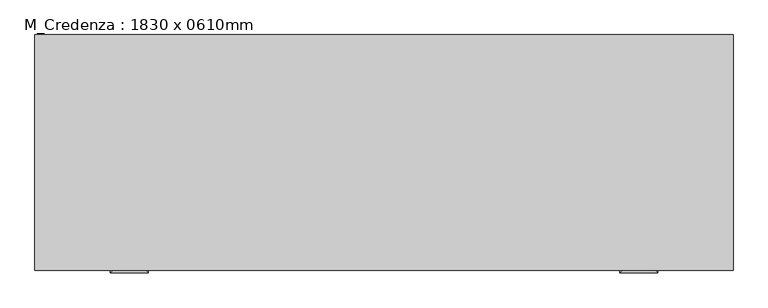
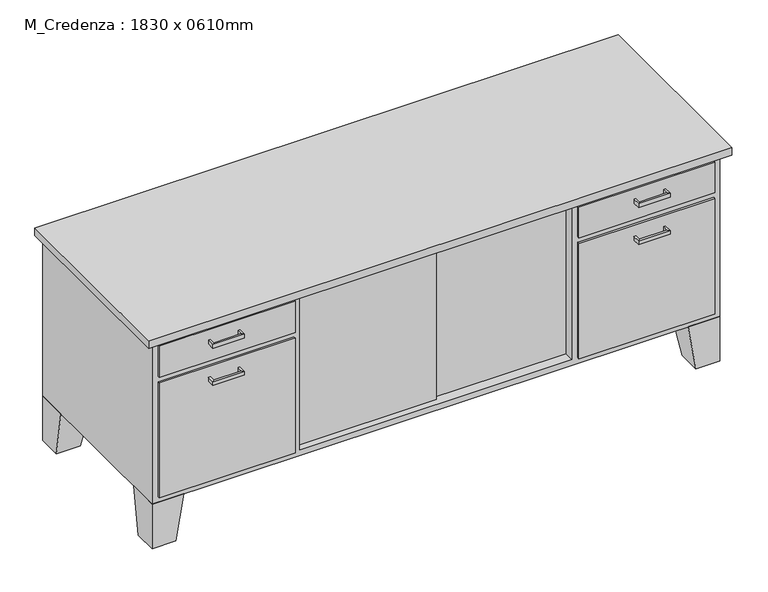
"""IFC4 building model written with IfcOpenShell, lengths in millimetres: furniture geometry, M_Credenza : 1830 x 0610mm."""

import ifcopenshell
import ifcopenshell.guid

model = None  # the IFC model being written
_history = None  # IfcOwnerHistory: only IFC2X3 demands one
_inside = {}  # id of a spatial element -> (the spatial element, [elements in it])
_under = {}  # id of a project, library or spatial element -> (it, [spatial elements below it])
_declared = {}  # id of a project -> (the project, [libraries it declares])
_typed = {}  # id of a type object -> (the type object, [elements of that type])
_made_of = {}  # id of a material, layer set ... -> (it, [elements and type objects made of it])


def new_model(schema):
    """Start an empty IFC model of exactly this schema.

    Asked for "IFC4X3", IfcOpenShell would pick the latest addendum, in which some entities
    have other attributes; the version numbers below select the first issue.
    IFC2X3 requires an IfcOwnerHistory on every rooted entity: one is made here for all.
    """
    global model, _history
    if schema == "IFC4X3":
        model = ifcopenshell.file(schema_version=(4, 3, 0, 0))
    else:
        model = ifcopenshell.file(schema=schema)
    _inside.clear()
    _under.clear()
    _declared.clear()
    _typed.clear()
    _made_of.clear()
    _history = None
    if model.schema == "IFC2X3":
        org = make("IfcOrganization", Name="unknown")
        user = make(
            "IfcPersonAndOrganization",
            ThePerson=make("IfcPerson", FamilyName="unknown"),
            TheOrganization=org,
        )
        app = make(
            "IfcApplication",
            ApplicationDeveloper=org,
            Version="unknown",
            ApplicationFullName="unknown",
            ApplicationIdentifier="unknown",
        )
        _history = make(
            "IfcOwnerHistory",
            OwningUser=user,
            OwningApplication=app,
            ChangeAction="ADDED",
            CreationDate=0,
        )
    return model


def make(cls, **values):
    """One entity of the class cls with the attributes given. An attribute that is None is left unset."""
    return model.create_entity(
        cls, **{name: value for name, value in values.items() if value is not None}
    )


def rooted(cls, **values):
    """An entity with a GlobalId (a new one), such as an element, a storey or a relation."""
    return make(cls, GlobalId=ifcopenshell.guid.new(), OwnerHistory=_history, **values)


def si_unit(unit_type, name, prefix=None):
    """IfcSIUnit, for example si_unit("LENGTHUNIT", "METRE", prefix="MILLI")."""
    return make("IfcSIUnit", UnitType=unit_type, Prefix=prefix, Name=name)


def assignment(units):
    """IfcUnitAssignment: the units of a project."""
    return None if units is None else make("IfcUnitAssignment", Units=units)


def point(xyz):
    """IfcCartesianPoint."""
    return None if xyz is None else make("IfcCartesianPoint", Coordinates=xyz)


def direction(xyz):
    """IfcDirection."""
    return None if xyz is None else make("IfcDirection", DirectionRatios=xyz)


def frame(location, z_axis=None, x_axis=None):
    """IfcAxis2Placement3D, a coordinate frame: its origin and axes. An axis left out is left unset."""
    return make(
        "IfcAxis2Placement3D",
        Location=point(location),
        Axis=direction(z_axis),
        RefDirection=direction(x_axis),
    )


def origin():
    """The frame at (0, 0, 0) with its axes left unset."""
    return frame((0.0, 0.0, 0.0))


def place(relative_to, where):
    """IfcLocalPlacement: puts the frame where relative to a parent placement (None: the world)."""
    return make(
        "IfcLocalPlacement", PlacementRelTo=relative_to, RelativePlacement=where
    )


def context(
    kind, dimensions, precision=None, world=None, true_north=None, identifier=None
):
    """IfcGeometricRepresentationContext, for example the 3D "Model" context."""
    return make(
        "IfcGeometricRepresentationContext",
        ContextIdentifier=identifier,
        ContextType=kind,
        CoordinateSpaceDimension=dimensions,
        Precision=precision,
        WorldCoordinateSystem=world,
        TrueNorth=true_north,
    )


def project(units=None, contexts=None):
    """IfcProject with its units and contexts."""
    return rooted(
        "IfcProject",
        Name="project",
        RepresentationContexts=contexts,
        UnitsInContext=assignment(units),
    )


def spatial(cls, under=None, at=None, **own):
    """A site, building, storey or space (cls), placed at a placement, below another one or the project."""
    s = rooted(cls, ObjectPlacement=at, **own)
    if under is not None:
        _under.setdefault(under.id(), (under, []))[1].append(s)
    return s


def polyline(points):
    """IfcPolyline through the points."""
    return make("IfcPolyline", Points=[point(p) for p in points])


def outline(outer, holes=None, kind="AREA"):
    """IfcArbitraryClosedProfileDef: a profile drawn as a closed curve; with holes, ...WithVoids."""
    if holes is None:
        return make("IfcArbitraryClosedProfileDef", ProfileType=kind, OuterCurve=outer)
    return make(
        "IfcArbitraryProfileDefWithVoids",
        ProfileType=kind,
        OuterCurve=outer,
        InnerCurves=holes,
    )


def extrude(swept, where, along, depth):
    """IfcExtrudedAreaSolid: the profile swept, set in the frame where, extruded along a direction by depth."""
    return make(
        "IfcExtrudedAreaSolid",
        SweptArea=swept,
        Position=where,
        ExtrudedDirection=direction(along),
        Depth=depth,
    )


def faces_of(points, faces, orient=None, outer=None):
    """IfcFace entities. A face is a list of loops; a loop is a list of indices into points, from 0.

    orient and outer hold one flag for each loop. By default every Orientation is true, the
    first loop of a face is its IfcFaceOuterBound and the others are IfcFaceBound.
    """
    made = []
    for i, loops in enumerate(faces):
        bounds = []
        for j, loop in enumerate(loops):
            is_outer = j == 0 if outer is None else outer[i][j]
            bounds.append(
                make(
                    "IfcFaceOuterBound" if is_outer else "IfcFaceBound",
                    Bound=make("IfcPolyLoop", Polygon=[points[k] for k in loop]),
                    Orientation=True if orient is None else orient[i][j],
                )
            )
        made.append(make("IfcFace", Bounds=bounds))
    return made


def faceted_brep(points, faces, orient=None, outer=None, voids=None):
    """IfcFacetedBrep: a solid bounded by flat faces; with voids (closed shells), ...WithVoids."""
    shared = [point(p) for p in points]
    hull = make("IfcClosedShell", CfsFaces=faces_of(shared, faces, orient, outer))
    if voids is None:
        return make("IfcFacetedBrep", Outer=hull)
    return make(
        "IfcFacetedBrepWithVoids",
        Outer=hull,
        Voids=[
            make(cls, CfsFaces=faces_of(shared, fs, o, b)) for cls, fs, o, b in voids
        ],
    )


def shape(context_of_items, identifier, shape_type, items):
    """IfcShapeRepresentation: the items that make up one representation, for example the "Body"."""
    return make(
        "IfcShapeRepresentation",
        ContextOfItems=context_of_items,
        RepresentationIdentifier=identifier,
        RepresentationType=shape_type,
        Items=items,
    )


def source(mapping_origin, context_of_items, identifier, shape_type, items):
    """IfcRepresentationMap: a shape defined once, which mapped items show again and again."""
    return make(
        "IfcRepresentationMap",
        MappingOrigin=mapping_origin,
        MappedRepresentation=shape(context_of_items, identifier, shape_type, items),
    )


def transform(
    local_origin,
    x_axis=None,
    y_axis=None,
    z_axis=None,
    scale=None,
    scale2=None,
    scale3=None,
    uniform=True,
):
    """IfcCartesianTransformationOperator3D, or its non-uniform kind. x_axis, y_axis, z_axis: its Axis1, 2, 3."""
    if uniform:
        return make(
            "IfcCartesianTransformationOperator3D",
            Axis1=direction(x_axis),
            Axis2=direction(y_axis),
            LocalOrigin=point(local_origin),
            Scale=scale,
            Axis3=direction(z_axis),
        )
    return make(
        "IfcCartesianTransformationOperator3DnonUniform",
        Axis1=direction(x_axis),
        Axis2=direction(y_axis),
        LocalOrigin=point(local_origin),
        Scale=scale,
        Axis3=direction(z_axis),
        Scale2=scale2,
        Scale3=scale3,
    )


def mapped(mapping_source, mapping_target):
    """IfcMappedItem: shows the shape of a source again, moved by a transform."""
    return make(
        "IfcMappedItem", MappingSource=mapping_source, MappingTarget=mapping_target
    )


def made_of(thing, what):
    """Note that an element or type object is made of a material, layer set ...; save() writes the relation."""
    if what is not None:
        _made_of.setdefault(what.id(), (what, []))[1].append(thing)
    return thing


def element(
    cls,
    number,
    at=None,
    inside=None,
    cuts=None,
    type_object=None,
    material=None,
    context=None,
    identifier="Body",
    shape_type=None,
    held_by="IfcProductDefinitionShape",
    body=None,
    shapes=None,
    **own,
):
    """One element of the class cls, such as IfcWall. Its Tag is "e" and its number.

    at: its placement. inside: the storey or other place that contains it. cuts: it is an
    opening in that element (IfcRelVoidsElement). A single representation is given by context,
    identifier, shape_type and body (its items); several are given by shapes. held_by: the class
    of the entity that holds the representations. save() writes the other relations.
    """
    e = rooted(cls, Tag="e%d" % number, ObjectPlacement=at, **own)
    if body is not None:
        shapes = [shape(context, identifier, shape_type, body)]
    if shapes is not None:
        e.Representation = make(held_by, Representations=shapes)
    if inside is not None:
        _inside.setdefault(inside.id(), (inside, []))[1].append(e)
    if cuts is not None:
        rooted(
            "IfcRelVoidsElement", RelatingBuildingElement=cuts, RelatedOpeningElement=e
        )
    if type_object is not None:
        _typed.setdefault(type_object.id(), (type_object, []))[1].append(e)
    return made_of(e, material)


def aggregate(whole, parts):
    """IfcRelAggregates: a whole, such as a stair, and the parts it consists of."""
    return rooted("IfcRelAggregates", RelatingObject=whole, RelatedObjects=parts)


def save(model, path):
    """Write the relations noted so far, then the file.

    IfcRelAggregates (storeys below a building ...), IfcRelContainedInSpatialStructure (elements
    in a storey), IfcRelDefinesByType, IfcRelAssociatesMaterial and IfcRelDeclares: one each for
    every whole, place, type object, material and project.
    """
    for whole, parts in _under.values():
        aggregate(whole, parts)
    for where, things in _inside.values():
        rooted(
            "IfcRelContainedInSpatialStructure",
            RelatedElements=things,
            RelatingStructure=where,
        )
    for kind, things in _typed.values():
        rooted("IfcRelDefinesByType", RelatedObjects=things, RelatingType=kind)
    for what, things in _made_of.values():
        rooted("IfcRelAssociatesMaterial", RelatedObjects=things, RelatingMaterial=what)
    for by, libraries in _declared.values():
        rooted("IfcRelDeclares", RelatingContext=by, RelatedDefinitions=libraries)
    model.write(path)


def m_credenza_1830_x_0610mm_1080a9db(model_context):
    return source(origin(), model_context, "Body", "SolidModel", [
        extrude(outline(polyline([(532.0023176, -267.0714583), (46.8442623, -267.0714583), (46.8442623, -254.7714583), (532.0023176, -254.7714583), (532.0023176, -267.0714583)])), frame((0.0, 0.0, 171.45), z_axis=(0.0, 0.0, 1.0), x_axis=(1.0, 0.0, 0.0)), (0.0, 0.0, 1.0), 518.1),
        extrude(outline(polyline([(73.6254475, -279.7714583), (-378.9057377, -279.7714583), (-378.9057377, -267.0714583), (73.6254475, -267.0714583), (73.6254475, -279.7714583)])), frame((0.0, 0.0, 171.45), z_axis=(0.0, 0.0, 1.0), x_axis=(1.0, 0.0, 0.0)), (0.0, 0.0, 1.0), 518.1),
        faceted_brep([(872.9442623, 309.5803279, 152.4), (872.9442623, 207.9803279, 152.4), (974.5442623, 207.9803279, 152.4), (974.5442623, 309.5803279, 152.4), (898.3442623, 309.5803279, 0.0), (974.5442623, 309.5803279, 0.0), (974.5442623, 233.3803279, 0.0), (898.3442623, 233.3803279, 0.0)], [[[0, 1, 2, 3]], [[4, 5, 6, 7]], [[4, 7, 1, 0]], [[7, 6, 2, 1]], [[6, 5, 3, 2]], [[5, 4, 0, 3]]]),
        extrude(outline(polyline([(955.4942623, -306.3696721), (517.0442623, -306.3696721), (517.0442623, -300.0196721), (955.4942623, -300.0196721), (955.4942623, -306.3696721)])), frame((0.0, 0.0, 584.2), z_axis=(0.0, 0.0, 1.0), x_axis=(1.0, 0.0, 0.0)), (0.0, 0.0, 1.0), 105.35),
        extrude(outline(polyline([(955.4942623, -306.3696721), (517.0442623, -306.3696721), (517.0442623, -300.0196721), (955.4942623, -300.0196721), (955.4942623, -306.3696721)])), frame((0.0, 0.0, 171.45), z_axis=(0.0, 0.0, 1.0), x_axis=(1.0, 0.0, 0.0)), (0.0, 0.0, 1.0), 393.7),
        extrude(outline(polyline([(-397.9557377, -306.7696721), (-836.4057377, -306.7696721), (-836.4057377, -300.4196721), (-397.9557377, -300.4196721), (-397.9557377, -306.7696721)])), frame((0.0, 0.0, 581.6), z_axis=(0.0, 0.0, 1.0), x_axis=(1.0, 0.0, 0.0)), (0.0, 0.0, 1.0), 107.95),
        extrude(outline(polyline([(-397.9557377, -306.7696721), (-836.4057377, -306.7696721), (-836.4057377, -300.4196721), (-397.9557377, -300.4196721), (-397.9557377, -306.7696721)])), frame((0.0, 0.0, 171.45), z_axis=(0.0, 0.0, 1.0), x_axis=(1.0, 0.0, 0.0)), (0.0, 0.0, 1.0), 391.1),
        faceted_brep([(-753.8557377, -300.4196721, 152.4), (-753.8557377, -198.8196721, 152.4), (-855.4557377, -198.8196721, 152.4), (-855.4557377, -300.4196721, 152.4), (-779.2557377, -300.4196721, 0.0), (-855.4557377, -300.4196721, 0.0), (-855.4557377, -224.2196721, 0.0), (-779.2557377, -224.2196721, 0.0)], [[[0, 1, 2, 3]], [[4, 5, 6, 7]], [[4, 7, 1, 0]], [[7, 6, 2, 1]], [[6, 5, 3, 2]], [[5, 4, 0, 3]]]),
        faceted_brep([(-753.8557377, 309.5803279, 152.4), (-855.4557377, 309.5803279, 152.4), (-855.4557377, 207.9803279, 152.4), (-753.8557377, 207.9803279, 152.4), (-779.2557377, 309.5803279, 0.0), (-779.2557377, 233.3803279, 0.0), (-855.4557377, 233.3803279, 0.0), (-855.4557377, 309.5803279, 0.0)], [[[0, 1, 2, 3]], [[4, 5, 6, 7]], [[4, 7, 1, 0]], [[7, 6, 2, 1]], [[6, 5, 3, 2]], [[5, 4, 0, 3]]]),
        faceted_brep([(872.9442623, -300.4196721, 152.4), (974.5442623, -300.4196721, 152.4), (974.5442623, -198.8196721, 152.4), (872.9442623, -198.8196721, 152.4), (898.3442623, -300.4196721, 0.0), (898.3442623, -224.2196721, 0.0), (974.5442623, -224.2196721, 0.0), (974.5442623, -300.4196721, 0.0)], [[[0, 1, 2, 3]], [[4, 5, 6, 7]], [[4, 7, 1, 0]], [[7, 6, 2, 1]], [[6, 5, 3, 2]], [[5, 4, 0, 3]]]),
        faceted_brep([(974.5442623, 309.5803279, 708.6), (-855.4557377, 309.5803279, 708.6), (-855.4557377, -300.4196721, 708.6), (974.5442623, -300.4196721, 708.6), (974.5442623, 309.5803279, 152.4), (974.5442623, -300.4196721, 152.4), (-855.4557377, -300.4196721, 152.4), (-855.4557377, 309.5803279, 152.4), (-378.9057377, -300.4196721, 689.55), (497.9942623, -300.4196721, 689.55), (497.9942623, -300.4196721, 171.45), (-378.9057377, -300.4196721, 171.45), (497.9942623, 290.3303279, 689.55), (-378.9057377, 290.3303279, 689.55), (-378.9057377, 290.3303279, 171.45), (497.9942623, 290.3303279, 171.45)], [[[0, 1, 2, 3]], [[4, 5, 6, 7]], [[1, 0, 4, 7]], [[2, 1, 7, 6]], [[3, 2, 6, 5], [8, 9, 10, 11]], [[0, 3, 5, 4]], [[12, 13, 14, 15]], [[13, 12, 9, 8]], [[14, 13, 8, 11]], [[15, 14, 11, 10]], [[12, 15, 10, 9]]]),
        extrude(outline(polyline([(999.9442623, 309.5803279), (999.9442623, -325.8196721), (-880.8557377, -325.8196721), (-880.8557377, 309.5803279), (999.9442623, 309.5803279)])), frame((0.0, 0.0, 708.6), z_axis=(0.0, 0.0, 1.0), x_axis=(1.0, 0.0, 0.0)), (0.0, 0.0, 1.0), 25.4),
        faceted_brep([(-671.1557377, -306.7696721, 527.05), (-671.1557377, -306.7696721, 514.35), (-677.5057377, -306.7696721, 514.35), (-677.5057377, -306.7696721, 527.05), (-671.1557377, -325.8196721, 527.05), (-671.1557377, -325.8196721, 514.35), (-677.5057377, -332.1696721, 514.35), (-677.5057377, -332.1696721, 527.05), (-582.2557377, -325.8196721, 527.05), (-582.2557377, -325.8196721, 514.35), (-575.9057377, -332.1696721, 514.35), (-575.9057377, -332.1696721, 527.05), (-582.2557377, -306.7696721, 527.05), (-575.9057377, -306.7696721, 527.05), (-575.9057377, -306.7696721, 514.35), (-582.2557377, -306.7696721, 514.35)], [[[0, 1, 2, 3]], [[1, 0, 4, 5]], [[2, 1, 5, 6]], [[3, 2, 6, 7]], [[0, 3, 7, 4]], [[5, 4, 8, 9]], [[6, 5, 9, 10]], [[7, 6, 10, 11]], [[4, 7, 11, 8]], [[12, 13, 14, 15]], [[9, 8, 12, 15]], [[10, 9, 15, 14]], [[11, 10, 14, 13]], [[8, 11, 13, 12]]]),
        faceted_brep([(-671.1557377, -306.7696721, 654.05), (-671.1557377, -306.7696721, 641.35), (-677.5057377, -306.7696721, 641.35), (-677.5057377, -306.7696721, 654.05), (-671.1557377, -325.8196721, 654.05), (-671.1557377, -325.8196721, 641.35), (-677.5057377, -332.1696721, 641.35), (-677.5057377, -332.1696721, 654.05), (-582.2557377, -325.8196721, 654.05), (-582.2557377, -325.8196721, 641.35), (-575.9057377, -332.1696721, 641.35), (-575.9057377, -332.1696721, 654.05), (-582.2557377, -306.7696721, 654.05), (-575.9057377, -306.7696721, 654.05), (-575.9057377, -306.7696721, 641.35), (-582.2557377, -306.7696721, 641.35)], [[[0, 1, 2, 3]], [[1, 0, 4, 5]], [[2, 1, 5, 6]], [[3, 2, 6, 7]], [[0, 3, 7, 4]], [[5, 4, 8, 9]], [[6, 5, 9, 10]], [[7, 6, 10, 11]], [[4, 7, 11, 8]], [[12, 13, 14, 15]], [[9, 8, 12, 15]], [[10, 9, 15, 14]], [[11, 10, 14, 13]], [[8, 11, 13, 12]]]),
        faceted_brep([(701.3442623, -306.7696721, 654.1373112), (701.3442623, -306.7696721, 641.4373112), (694.9942623, -306.7696721, 641.4373112), (694.9942623, -306.7696721, 654.1373112), (701.3442623, -325.8196721, 654.1373112), (701.3442623, -325.8196721, 641.4373112), (694.9942623, -332.1696721, 641.4373112), (694.9942623, -332.1696721, 654.1373112), (790.2442623, -325.8196721, 654.1373112), (790.2442623, -325.8196721, 641.4373112), (796.5942623, -332.1696721, 641.4373112), (796.5942623, -332.1696721, 654.1373112), (790.2442623, -306.7696721, 654.1373112), (796.5942623, -306.7696721, 654.1373112), (796.5942623, -306.7696721, 641.4373112), (790.2442623, -306.7696721, 641.4373112)], [[[0, 1, 2, 3]], [[1, 0, 4, 5]], [[2, 1, 5, 6]], [[3, 2, 6, 7]], [[0, 3, 7, 4]], [[5, 4, 8, 9]], [[6, 5, 9, 10]], [[7, 6, 10, 11]], [[4, 7, 11, 8]], [[12, 13, 14, 15]], [[9, 8, 12, 15]], [[10, 9, 15, 14]], [[11, 10, 14, 13]], [[8, 11, 13, 12]]]),
        faceted_brep([(701.3442623, -306.7696721, 527.05), (701.3442623, -306.7696721, 514.35), (694.9942623, -306.7696721, 514.35), (694.9942623, -306.7696721, 527.05), (701.3442623, -325.8196721, 527.05), (701.3442623, -325.8196721, 514.35), (694.9942623, -332.1696721, 514.35), (694.9942623, -332.1696721, 527.05), (790.2442623, -325.8196721, 527.05), (790.2442623, -325.8196721, 514.35), (796.5942623, -332.1696721, 514.35), (796.5942623, -332.1696721, 527.05), (790.2442623, -306.7696721, 527.05), (796.5942623, -306.7696721, 527.05), (796.5942623, -306.7696721, 514.35), (790.2442623, -306.7696721, 514.35)], [[[0, 1, 2, 3]], [[1, 0, 4, 5]], [[2, 1, 5, 6]], [[3, 2, 6, 7]], [[0, 3, 7, 4]], [[5, 4, 8, 9]], [[6, 5, 9, 10]], [[7, 6, 10, 11]], [[4, 7, 11, 8]], [[12, 13, 14, 15]], [[9, 8, 12, 15]], [[10, 9, 15, 14]], [[11, 10, 14, 13]], [[8, 11, 13, 12]]]),
    ])


if __name__ == "__main__":
    model = new_model("IFC4")
    model_context = context("Model", 3, world=origin())
    ifc_project = project(units=[si_unit("LENGTHUNIT", "METRE", prefix="MILLI")], contexts=[model_context])
    site = spatial("IfcSite", under=ifc_project)
    building = spatial("IfcBuilding", under=site)
    placement = place(None, origin())
    m_credenza_1830_x_0610mm_shape = m_credenza_1830_x_0610mm_1080a9db(model_context)
    element("IfcFurniture", 1, ObjectType="M_Credenza : 1830 x 0610mm", at=placement, inside=building, context=model_context, shape_type="MappedRepresentation", body=[
        mapped(m_credenza_1830_x_0610mm_shape, transform((0.0, 0.0, 0.0), x_axis=(1.0, 0.0, 0.0), y_axis=(0.0, 1.0, 0.0), z_axis=(0.0, 0.0, 1.0))),
    ])
    save(model, "model.ifc")

# Revit data of these elements
# Project information
#   Organization Name = "André Wisén"
#   Organization Description = "https://andrewisen.se/"
#   Building Name = "https://andrewisen.se/"
#   Author = "André Wisén"
#   Project Issue Date = "Issue Date"
#   Project Status = "Project  Status"
#   Client Name = "Owner"
#   Project Address = "## Street\nCity, State  Zip"
#   Project Name = "Project Name"
#   Project Number = "0001"
# Type "M_Credenza : 1830 x 0610mm"
#   Depth = 610 mm
#   Height = 734 mm
#   Width = 1830 mm
#   Desk-Body = Laminate, Ivory, Matte
#   Handle/Leg Material = Steel, Chrome Plated
#   Top Material = Cherry
#   Default Elevation = 0
# Element 1 (IfcFurniture, "M_Credenza : 1830 x 0610mm")
#   Materials on its faces: "Steel, Chrome Plated", "Laminate, Ivory, Matte", "Cherry"
# Materials
#   "Laminate, Ivory, Matte": class "Plastic", colour RGB 247 247 239, transparency 0, Description = "Plastic Laminate - Ivory, Matte", Cost = 0
#   "Steel, Chrome Plated": class "Metal", colour RGB 17 17 17, transparency 0, Description = "Chromiuim plated steel", Cost = 0
#   "Cherry": class "Wood", colour RGB 226 177 128, transparency 0, Description = "Prunus Serotina", Cost = 0
